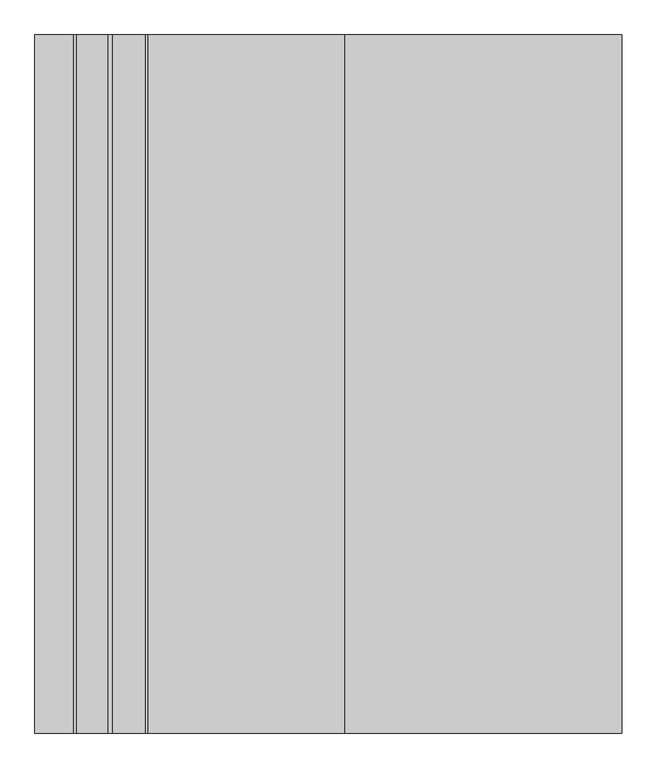
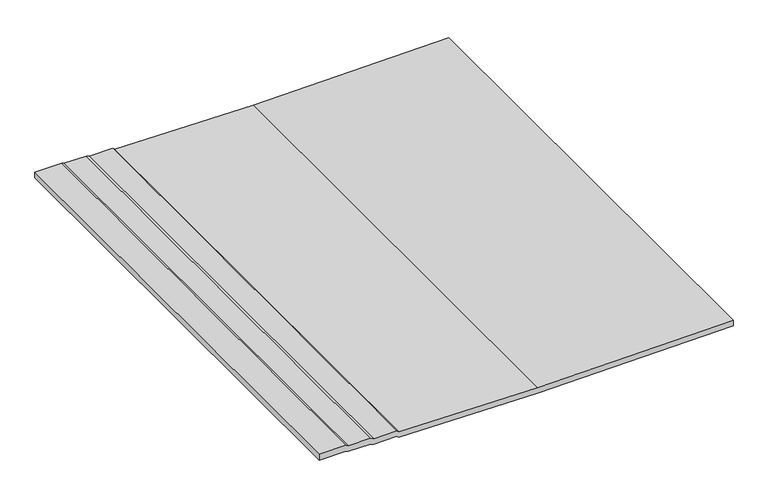
"""IFC4 building model written with IfcOpenShell, lengths in millimetres: proxy geometry, GRAVEL BALLAST2:GRAVEL BALLAST004:295726 : GRAVEL BALLAST2:GRAVEL BALLAST004:295726."""

from ifc_helpers import new_model, si_unit, frame, origin, place, context, project, spatial, polyline, outline, extrude, source, transform, mapped, element, save


def generic_models_ae22e0ce(model_context):
    return source(origin(), model_context, "Body", "SweptSolid", [
        extrude(outline(polyline([(40274.2359464, 1995.1433186), (40274.2359464, 2104.6428303), (40269.9546964, 2113.3532795), (40269.9546964, 2203.9401936), (40264.2272344, 2216.7848329), (40265.8726651, 2310.7365803), (40258.4625089, 2319.0100178), (40250.2437589, 2882.0804523), (40261.546875, 3677.8183121), (40286.2851563, 3677.8183121), (40274.9820402, 2882.0804523), (40283.2007902, 2319.0100178), (40290.6109464, 2310.7365803), (40288.9655157, 2216.7848329), (40294.6929777, 2203.9401936), (40294.6929777, 2113.3532795), (40298.9742277, 2104.6428303), (40298.9742277, 1995.1433186), (40274.2359464, 1995.1433186)])), frame((0.0, 1278.3325411, 0.0), z_axis=(0.0, 1.0, 0.0), x_axis=(0.0, 0.0, 1.0)), (0.0, 0.0, 1.0), 2000.0),
    ])


if __name__ == "__main__":
    model = new_model("IFC4")
    model_context = context("Model", 3, world=origin())
    ifc_project = project(units=[si_unit("LENGTHUNIT", "METRE", prefix="MILLI")], contexts=[model_context])
    site = spatial("IfcSite", under=ifc_project)
    building = spatial("IfcBuilding", under=site)
    placement = place(None, origin())
    generic_models_shape = generic_models_ae22e0ce(model_context)
    element("IfcBuildingElementProxy", 1, Name="GRAVEL BALLAST2:GRAVEL BALLAST004:295726 : GRAVEL BALLAST2:GRAVEL BALLAST004:295726", ObjectType="GRAVEL BALLAST2:GRAVEL BALLAST004:295726 : GRAVEL BALLAST2:GRAVEL BALLAST004:295726", at=placement, inside=building, context=model_context, shape_type="MappedRepresentation", body=[
        mapped(generic_models_shape, transform((0.0, 0.0, 0.0), x_axis=(1.0, 0.0, 0.0), y_axis=(0.0, 1.0, 0.0), z_axis=(0.0, 0.0, 1.0))),
    ])
    save(model, "model.ifc")

# Revit data of these elements
# Type "GRAVEL BALLAST2:GRAVEL BALLAST004:295726 : GRAVEL BALLAST2:GRAVEL BALLAST004:295726"
#   NameOverride = "GRAVEL BALLAST2:GRAVEL BALLAST004:295726"
#   ObjectTypeOverride = "GRAVEL BALLAST2:GRAVEL BALLAST004"
#   Reference = "GRAVEL BALLAST004"
#   Category = "Generic Models"
#   Tag = "295726"
# Element 1 (IfcBuildingElementProxy, "GRAVEL BALLAST2:GRAVEL BALLAST004:295726 : GRAVEL BALLAST2:GRAVEL BALLAST004:295726")
#   Materials on its faces: "GRAVEL BALLAST"
# Materials
#   "GRAVEL BALLAST": class "Unassigned", colour RGB 128 128 128, transparency 0, Cost = 0
